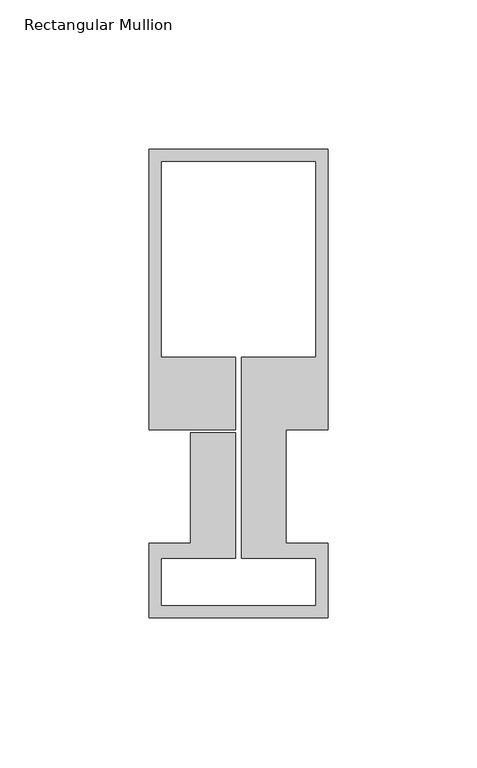
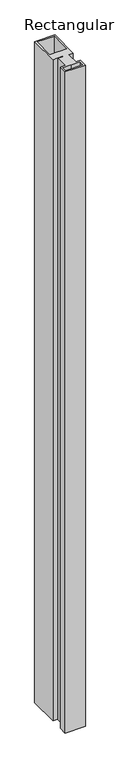
"""IFC4 building model written with IfcOpenShell, lengths in millimetres: member geometry, Rectangular Mullion : Schueco_FWS-60-SI_Mull_CovCap-20mm_Mull-85mm."""

from ifc_helpers import new_model, si_unit, frame, origin, place, context, project, spatial, polyline, outline, extrude, source, transform, mapped, element, save


def rectangular_mullion_017c49a8(model_context):
    return source(origin(), model_context, "Body", "SweptSolid", [
        extrude(outline(polyline([(30.0, 132.0), (30.0, 38.0), (16.0, 38.0), (16.0, -0.1), (30.0, -0.1), (30.0, -25.0), (-30.0, -25.0), (-30.0, -0.1), (-16.0, -0.1), (-16.0, 37.0), (-1.0, 37.0), (-1.0, -5.0), (-26.0, -5.0), (-26.0, -21.0), (26.0, -21.0), (26.0, -5.0), (1.0, -5.0), (1.0, 62.3), (26.0, 62.3), (26.0, 128.0), (-26.0, 128.0), (-26.0, 62.3), (-1.0, 62.3), (-1.0, 38.0), (-30.0, 38.0), (-30.0, 132.0), (30.0, 132.0)])), frame((0.0, 0.0, -2080.0), z_axis=(0.0, 0.0, 1.0), x_axis=(1.0, 0.0, 0.0)), (0.0, 0.0, 1.0), 2080.0),
    ])


if __name__ == "__main__":
    model = new_model("IFC4")
    model_context = context("Model", 3, world=origin())
    ifc_project = project(units=[si_unit("LENGTHUNIT", "METRE", prefix="MILLI")], contexts=[model_context])
    site = spatial("IfcSite", under=ifc_project)
    building = spatial("IfcBuilding", under=site)
    placement = place(None, origin())
    rectangular_mullion_shape = rectangular_mullion_017c49a8(model_context)
    element("IfcMember", 1, ObjectType="Rectangular Mullion : Schueco_FWS-60-SI_Mull_CovCap-20mm_Mull-85mm", at=placement, inside=building, context=model_context, shape_type="MappedRepresentation", body=[
        mapped(rectangular_mullion_shape, transform((0.0, 0.0, 0.0), x_axis=(1.0, 0.0, 0.0), y_axis=(0.0, 1.0, 0.0), z_axis=(0.0, 0.0, 1.0))),
    ])
    save(model, "model.ifc")

# Revit data of these elements
# Project information
#   Project Issue Date = "09.2017"
#   Project Status = "Project  Status"
#   Client Name = "Owner"
#   Project Address = "## Street\nCity, State  Zip"
#   Project Name = "Project Name"
#   Project Number = "0001"
# Type "Rectangular Mullion : Schueco_FWS-60-SI_Mull_CovCap-20mm_Mull-85mm"
#   Model = "FWS 60.SI"
#   Manufacturer = "Schueco International KG"
#   Type Comments = "Mullion"
#   Schueco thermal insulation standard = "Suitable for passive houses"
#   Burglar resistance = "RC 3"
#   Thermal insulation = "to 0.70 W/(m²K)"
#   built-in parameter 1007322 = 0.515092 (stored number, unit not read)
#   built-in parameter 1007321 = 0.0524934 (stored number, unit not read)
#   built-in parameter 1007320 = 0.0524934 (stored number, unit not read)
# Element 1 (IfcMember, "Rectangular Mullion : Schueco_FWS-60-SI_Mull_CovCap-20mm_Mull-85mm")
#   Materials on its faces: "Alu"
# Materials
#   "Alu": class "Glas", colour RGB 140 140 140, transparency 0
